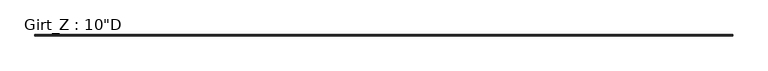
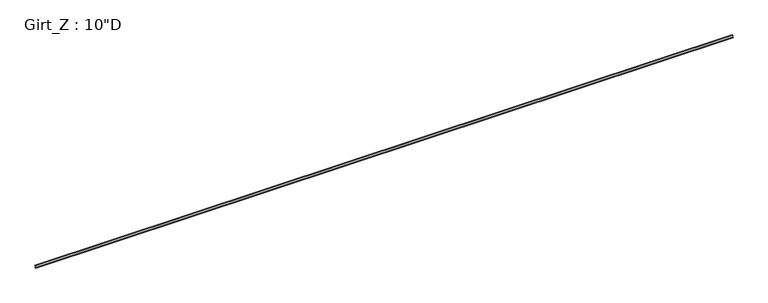
"""IFC4 building model written with IfcOpenShell, lengths in millimetres: beam geometry."""

from ifc_helpers import new_model, si_unit, point, frame, frame_2d, origin, place, context, project, spatial, polyline, circle_curve, trimmed, segment, composite_curve, outline, extrude, source, transform, mapped, element, save


def beam_bf61a610(model_context):
    return source(origin(), model_context, "Body", "SweptSolid", [
        extrude(outline(composite_curve([segment(polyline([(77.9859375, 127.0), (90.2310415, 112.4068534), (88.1028742, 110.621109), (76.6904765, 124.221875), (3.3005807, 124.221875)]), True, "CONTINUOUS"), segment(trimmed(circle_curve(frame_2d((3.3741066, 122.2381931)), 1.9850441), [point((3.3005807, 124.221875))], [point((1.3890625, 122.2381931))], True, "CARTESIAN"), True, "CONTINUOUS"), segment(polyline([(1.3890625, 122.2381931), (1.3890625, -127.0), (-84.3359375, -127.0), (-96.5810415, -112.4068534), (-94.4528742, -110.621109), (-83.0404765, -124.221875), (-3.2694106, -124.221875)]), True, "CONTINUOUS"), segment(trimmed(circle_curve(frame_2d((-3.3748024, -122.2389339)), 1.9857399), [point((-3.2694106, -124.221875))], [point((-1.3890625, -122.2389339))], True, "CARTESIAN"), True, "CONTINUOUS"), segment(polyline([(-1.3890625, -122.2389339), (-1.3890625, 122.2375)]), True, "CONTINUOUS"), segment(trimmed(circle_curve(frame_2d((3.3734375, 122.2375)), 4.7625), [point((-1.3890625, 122.2375))], [point((3.3734375, 127.0))], False, "CARTESIAN"), True, "CONTINUOUS"), segment(polyline([(3.3734375, 127.0), (77.9859375, 127.0)]), True, "CONTINUOUS")], self_intersect=False)), frame((-44283.1884767, 0.0, 0.0), z_axis=(1.0, 0.0, 0.0), x_axis=(0.0, 1.0, 0.0)), (0.0, 0.0, 1.0), 88566.3769533),
    ])


if __name__ == "__main__":
    model = new_model("IFC4")
    model_context = context("Model", 3, world=origin())
    ifc_project = project(units=[si_unit("LENGTHUNIT", "METRE", prefix="MILLI")], contexts=[model_context])
    site = spatial("IfcSite", under=ifc_project)
    building = spatial("IfcBuilding", under=site)
    placement = place(None, origin())
    beam_shape = beam_bf61a610(model_context)
    element("IfcBeam", 1, ObjectType="Girt_Z : 10\"D", at=placement, inside=building, context=model_context, shape_type="MappedRepresentation", body=[
        mapped(beam_shape, transform((0.0, 0.0, 0.0), x_axis=(1.0, 0.0, 0.0), y_axis=(0.0, 1.0, 0.0), z_axis=(0.0, 0.0, 1.0))),
    ])
    save(model, "model.ifc")

# Revit data of these elements
# Type "Girt_Z : 10\"D"
#   half leg = 0' - 1 11/16"
#   Web_Thickness = 0' - 0 7/64"
#   Length [instance default] = 10' - 0"
#   Leg_2 = 0' - 3 3/8"
#   Leg_1 = 0' - 3 1/8"
#   Height = 0' - 10"
#   Structural Material [instance default] = none
# Element 1 (IfcBeam, "Girt_Z : 10\"D")
#   Structural Material = STRUCTURAL STEEL - SEE STRUCT. DWGS
#   Materials on its faces: "STRUCTURAL STEEL - SEE STRUCT. DWGS"
# Materials
#   "STRUCTURAL STEEL - SEE STRUCT. DWGS": class "Metal", colour RGB 137 146 153, transparency 0, Description = "Steel, mill finish", Cost = 0
